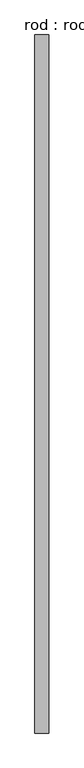
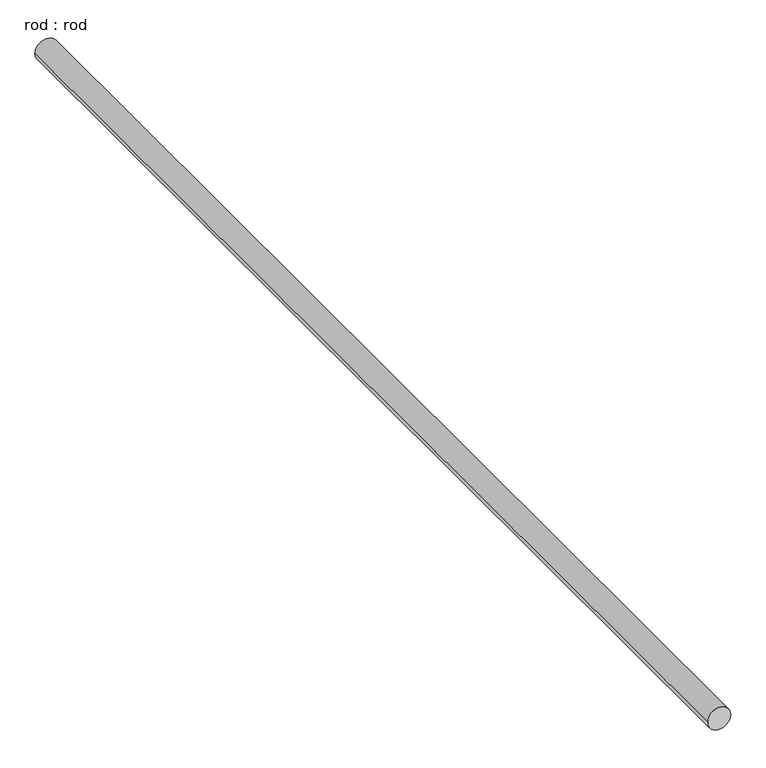
"""IFC4 building model written with IfcOpenShell, lengths in millimetres: proxy geometry, rod : rod."""

from ifc_helpers import new_model, si_unit, point, frame, frame_2d, origin, place, context, project, spatial, circle_curve, trimmed, segment, composite_curve, outline, extrude, source, transform, mapped, element, save


def rod_rod_446b7bbb(model_context):
    return source(origin(), model_context, "Body", "SweptSolid", [
        extrude(outline(composite_curve([segment(trimmed(circle_curve(frame_2d((0.0108462, 0.0)), 200.0), [point((0.0108462, 200.0))], [point((0.0108462, -200.0))], False, "CARTESIAN"), True, "CONTINUOUS"), segment(trimmed(circle_curve(frame_2d((0.0108462, 0.0)), 200.0), [point((0.0108462, -200.0))], [point((0.0108462, 200.0))], False, "CARTESIAN"), True, "CONTINUOUS")], self_intersect=False)), frame((0.0, -6005.4856704, 0.0), z_axis=(0.0, 1.0, 0.0), x_axis=(0.0, 0.0, 1.0)), (0.0, 0.0, 1.0), 20196.4285714),
    ])


if __name__ == "__main__":
    model = new_model("IFC4")
    model_context = context("Model", 3, world=origin())
    ifc_project = project(units=[si_unit("LENGTHUNIT", "METRE", prefix="MILLI")], contexts=[model_context])
    site = spatial("IfcSite", under=ifc_project)
    building = spatial("IfcBuilding", under=site)
    placement = place(None, origin())
    rod_rod_shape = rod_rod_446b7bbb(model_context)
    element("IfcBuildingElementProxy", 1, Name="rod : rod", ObjectType="rod : rod", at=placement, inside=building, context=model_context, shape_type="MappedRepresentation", body=[
        mapped(rod_rod_shape, transform((0.0, 0.0, 0.0), x_axis=(1.0, 0.0, 0.0), y_axis=(0.0, 1.0, 0.0), z_axis=(0.0, 0.0, 1.0))),
    ])
    save(model, "model.ifc")

# Revit data of these elements
# Type "rod : rod"
#   Default Elevation = 0
